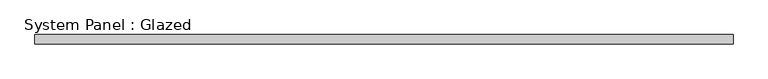
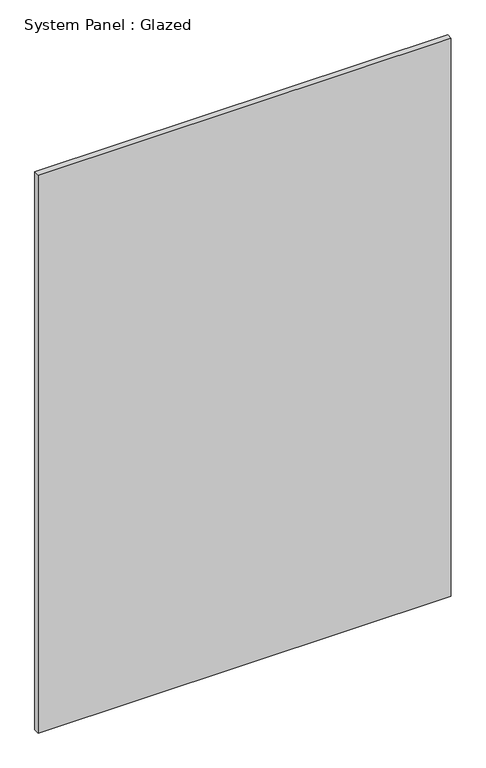
"""IFC4 building model written with IfcOpenShell, lengths in millimetres: plate geometry, System Panel : Glazed."""

from ifc_helpers import new_model, si_unit, origin, origin_with_axes, place, context, project, spatial, polyline, outline, extrude, source, transform, mapped, element, save


def system_panel_glazed_9cf86430(model_context):
    return source(origin(), model_context, "Body", "SweptSolid", [
        extrude(outline(polyline([(919.4444444, 24.5), (-919.4444444, 24.5), (-919.4444444, 49.5), (919.4444444, 49.5), (919.4444444, 24.5)])), origin_with_axes(), (0.0, 0.0, 1.0), 2625.0),
    ])


if __name__ == "__main__":
    model = new_model("IFC4")
    model_context = context("Model", 3, world=origin())
    ifc_project = project(units=[si_unit("LENGTHUNIT", "METRE", prefix="MILLI")], contexts=[model_context])
    site = spatial("IfcSite", under=ifc_project)
    building = spatial("IfcBuilding", under=site)
    placement = place(None, origin())
    system_panel_glazed_shape = system_panel_glazed_9cf86430(model_context)
    element("IfcPlate", 1, ObjectType="System Panel : Glazed", at=placement, inside=building, context=model_context, shape_type="MappedRepresentation", body=[
        mapped(system_panel_glazed_shape, transform((0.0, 0.0, 0.0), x_axis=(1.0, 0.0, 0.0), y_axis=(0.0, 1.0, 0.0), z_axis=(0.0, 0.0, 1.0))),
    ])
    save(model, "model.ifc")

# Revit data of these elements
# Element 1 (IfcPlate, "System Panel : Glazed")
#   Materials on its faces: "Glass"
# Materials
#   "Glass": class "Glass", colour RGB 0 128 192, transparency 0.9
